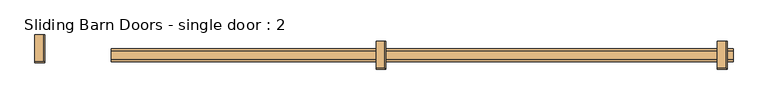
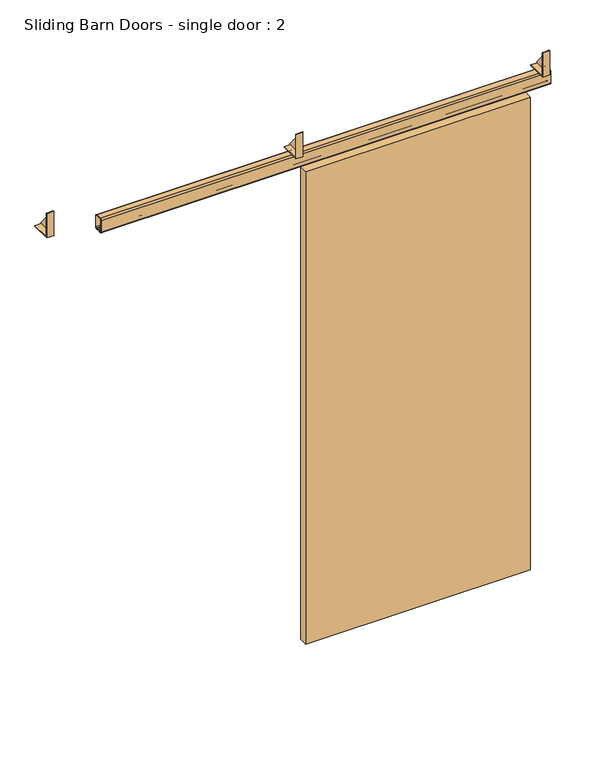
"""IFC4 building model written with IfcOpenShell, lengths in millimetres: door geometry, Sliding Barn Doors - single door : 2."""

from ifc_helpers import new_model, si_unit, point, frame, frame_2d, origin, place, context, project, spatial, polyline, circle_curve, trimmed, segment, composite_curve, outline, extrude, source, transform, mapped, element, save


def sliding_barn_doors_single_door_2_0560d3d1(model_context):
    return source(origin(), model_context, "Body", "SweptSolid", [
        extrude(outline(polyline([(158.75, 2152.65), (158.75, 2146.3), (79.375, 2146.3), (79.375, 2247.773), (158.75, 2152.65)])), frame((-1487.5371094, 0.0, 0.0), z_axis=(1.0, 0.0, 0.0), x_axis=(0.0, 1.0, 0.0)), (0.0, 0.0, 1.0), 3.175),
        extrude(outline(polyline([(76.2, 2143.125), (76.2, 2247.773), (79.375, 2247.773), (79.375, 2146.3), (158.75, 2146.3), (158.75, 2143.125), (76.2, 2143.125)])), frame((-1512.8378906, 0.0, 0.0), z_axis=(1.0, 0.0, 0.0), x_axis=(0.0, 1.0, 0.0)), (0.0, 0.0, 1.0), 28.4757812),
        extrude(outline(polyline([(139.7, 2152.65), (139.7, 2146.3), (60.325, 2146.3), (60.325, 2247.773), (139.7, 2152.65)])), frame((-484.2371094, 0.0, 0.0), z_axis=(1.0, 0.0, 0.0), x_axis=(0.0, 1.0, 0.0)), (0.0, 0.0, 1.0), 3.175),
        extrude(outline(polyline([(57.15, 2143.125), (57.15, 2247.773), (60.325, 2247.773), (60.325, 2146.3), (139.7, 2146.3), (139.7, 2143.125), (57.15, 2143.125)])), frame((-509.5378906, 0.0, 0.0), z_axis=(1.0, 0.0, 0.0), x_axis=(0.0, 1.0, 0.0)), (0.0, 0.0, 1.0), 28.4757813),
        extrude(outline(polyline([(139.7, 2152.65), (139.7, 2146.3), (60.325, 2146.3), (60.325, 2247.773), (139.7, 2152.65)])), frame((519.0628906, 0.0, 0.0), z_axis=(1.0, 0.0, 0.0), x_axis=(0.0, 1.0, 0.0)), (0.0, 0.0, 1.0), 3.175),
        extrude(outline(polyline([(57.15, 2143.125), (57.15, 2247.773), (60.325, 2247.773), (60.325, 2146.3), (139.7, 2146.3), (139.7, 2143.125), (57.15, 2143.125)])), frame((493.7621094, 0.0, 0.0), z_axis=(1.0, 0.0, 0.0), x_axis=(0.0, 1.0, 0.0)), (0.0, 0.0, 1.0), 28.4757813),
        extrude(outline(polyline([(-355.854, 117.475), (-304.546, 117.475), (-304.546, 114.3), (-355.854, 114.3), (-355.854, 117.475)])), frame((0.0, 0.0, 1889.252), z_axis=(0.0, 0.0, 1.0), x_axis=(1.0, 0.0, 0.0)), (0.0, 0.0, 1.0), 168.148),
        extrude(outline(polyline([(304.546, 117.475), (355.854, 117.475), (355.854, 114.3), (304.546, 114.3), (304.546, 117.475)])), frame((0.0, 0.0, 1889.252), z_axis=(0.0, 0.0, 1.0), x_axis=(1.0, 0.0, 0.0)), (0.0, 0.0, 1.0), 168.148),
        extrude(outline(polyline([(-457.2, 114.3), (457.2, 114.3), (457.2, 79.375), (-457.2, 79.375), (-457.2, 114.3)])), frame((0.0, 0.0, 25.4), z_axis=(0.0, 0.0, 1.0), x_axis=(1.0, 0.0, 0.0)), (0.0, 0.0, 1.0), 2032.0),
        extrude(outline(composite_curve([segment(polyline([(85.725, 2143.125), (111.252, 2143.125)]), True, "CONTINUOUS"), segment(trimmed(circle_curve(frame_2d((111.252, 2136.775)), 6.35), [point((111.252, 2143.125))], [point((117.602, 2136.775))], False, "CARTESIAN"), True, "CONTINUOUS"), segment(polyline([(117.602, 2136.775), (117.602, 2088.515)]), True, "CONTINUOUS"), segment(trimmed(circle_curve(frame_2d((111.252, 2088.515)), 6.35), [point((117.602, 2088.515))], [point((111.252, 2082.165))], False, "CARTESIAN"), True, "CONTINUOUS"), segment(polyline([(111.252, 2082.165), (105.8433147, 2082.165)]), True, "CONTINUOUS"), segment(trimmed(circle_curve(frame_2d((105.8433147, 2083.7525)), 1.5875), [point((105.8433147, 2082.165))], [point((104.2849816, 2083.4495907))], False, "CARTESIAN"), True, "CONTINUOUS"), segment(polyline([(104.2849816, 2083.4495907), (102.8594659, 2090.7832331), (104.3756029, 2090.7832331), (105.7615251, 2083.6532812), (111.252, 2083.6532812)]), True, "CONTINUOUS"), segment(trimmed(circle_curve(frame_2d((111.252, 2088.515)), 4.8617187), [point((111.252, 2083.6532812))], [point((116.1137188, 2088.515))], True, "CARTESIAN"), True, "CONTINUOUS"), segment(polyline([(116.1137188, 2088.515), (116.1137188, 2136.775)]), True, "CONTINUOUS"), segment(trimmed(circle_curve(frame_2d((111.252, 2136.775)), 4.8617187), [point((116.1137188, 2136.775))], [point((111.252, 2141.6367187))], True, "CARTESIAN"), True, "CONTINUOUS"), segment(polyline([(111.252, 2141.6367187), (85.725, 2141.6367187)]), True, "CONTINUOUS"), segment(trimmed(circle_curve(frame_2d((85.725, 2136.775)), 4.8617187), [point((85.725, 2141.6367187))], [point((80.8632813, 2136.775))], True, "CARTESIAN"), True, "CONTINUOUS"), segment(polyline([(80.8632813, 2136.775), (80.8632813, 2088.515)]), True, "CONTINUOUS"), segment(trimmed(circle_curve(frame_2d((85.725, 2088.515)), 4.8617187), [point((80.8632813, 2088.515))], [point((85.725, 2083.6532812))], True, "CARTESIAN"), True, "CONTINUOUS"), segment(polyline([(85.725, 2083.6532812), (91.2154749, 2083.6532812), (92.6013971, 2090.7832331), (94.1175341, 2090.7832331), (92.6920184, 2083.4495907)]), True, "CONTINUOUS"), segment(trimmed(circle_curve(frame_2d((91.1336853, 2083.7525)), 1.5875), [point((92.6920184, 2083.4495907))], [point((91.1336853, 2082.165))], False, "CARTESIAN"), True, "CONTINUOUS"), segment(polyline([(91.1336853, 2082.165), (85.725, 2082.165)]), True, "CONTINUOUS"), segment(trimmed(circle_curve(frame_2d((85.725, 2088.515)), 6.35), [point((85.725, 2082.165))], [point((79.375, 2088.515))], False, "CARTESIAN"), True, "CONTINUOUS"), segment(polyline([(79.375, 2088.515), (79.375, 2136.775)]), True, "CONTINUOUS"), segment(trimmed(circle_curve(frame_2d((85.725, 2136.775)), 6.35), [point((79.375, 2136.775))], [point((85.725, 2143.125))], False, "CARTESIAN"), True, "CONTINUOUS")], self_intersect=False)), frame((-1289.05, 0.0, 0.0), z_axis=(1.0, 0.0, 0.0), x_axis=(0.0, 1.0, 0.0)), (0.0, 0.0, 1.0), 1828.8),
    ])


if __name__ == "__main__":
    model = new_model("IFC4")
    model_context = context("Model", 3, world=origin())
    ifc_project = project(units=[si_unit("LENGTHUNIT", "METRE", prefix="MILLI")], contexts=[model_context])
    site = spatial("IfcSite", under=ifc_project)
    building = spatial("IfcBuilding", under=site)
    placement = place(None, origin())
    sliding_barn_doors_single_door_2_shape = sliding_barn_doors_single_door_2_0560d3d1(model_context)
    element("IfcDoor", 1, ObjectType="Sliding Barn Doors - single door : 2", at=placement, inside=building, context=model_context, shape_type="MappedRepresentation", body=[
        mapped(sliding_barn_doors_single_door_2_shape, transform((0.0, 0.0, 0.0), x_axis=(1.0, 0.0, 0.0), y_axis=(0.0, 1.0, 0.0), z_axis=(0.0, 0.0, 1.0))),
    ])
    save(model, "model.ifc")

# Revit data of these elements
# Type "Sliding Barn Doors - single door : 2"
#   Type Mark = "62"
#   OD_DS_Door_Material = "T.B.D."
#   OD_DS_Door_Type = "SLIDER"
#   OD_DS_Lockset = "-"
#   Analytic Construction = "<None>"
#   rail_overlap_left = 0' - 5 1/4"
#   rail_length = 6' - 0"
#   overlap_left = 0' - 2"
#   overlap = 0' - 0"
#   bracket_right = 3' - 7"
#   bracket_left = 0' - 4"
#   Thickness = 0' - 1 3/8"
#   Panel Width = 3' - 0"
#   Panel Height = 6' - 8"
#   Gap 2 = 0' - 0 1/2"
#   Gap 1 = 0' - 0 7/8"
#   Frame Projection Ext. = 0' - 1"
#   Frame Projection Int. = 0' - 1"
#   Frame Width = 0' - 3"
#   Height = 6' - 4"
#   Width = 2' - 8"
#   Bracket_offset = 0' - 5"
#   Door_4 = no
#   Door_3 = no
#   Hardware Material = Metal - Aluminum
#   Door Material = Closet_1
#   Function = (empty or 0)
#   Wall Closure = (empty or 0)
# Element 1 (IfcDoor, "Sliding Barn Doors - single door : 2")
#   Materials on its faces: "Metal - Aluminum", "Closet_1"
# Materials
#   "Metal - Aluminum": class "Metal", colour RGB 247 247 247, transparency 0
#   "Closet_1": class "Paint", colour RGB 200 194 183, transparency 0, Cost = 0
